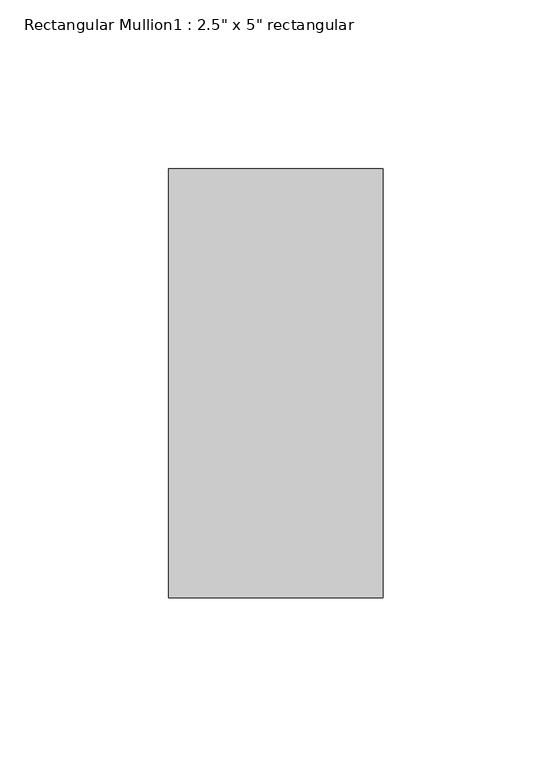
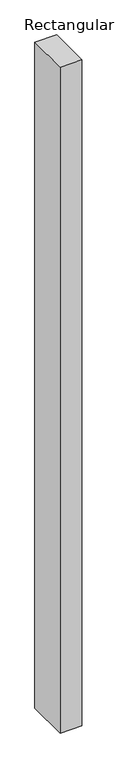
"""IFC4 building model written with IfcOpenShell, lengths in millimetres: member geometry."""

from ifc_helpers import new_model, si_unit, frame, origin, place, context, project, spatial, polyline, outline, extrude, source, transform, mapped, element, save


def member_60f5540e(model_context):
    return source(origin(), model_context, "Body", "SweptSolid", [
        extrude(outline(polyline([(0.0, 63.5), (0.0, -63.5), (-63.5, -63.5), (-63.5, 63.5), (0.0, 63.5)])), frame((0.0, 0.0, -2053.1666667), z_axis=(0.0, 0.0, 1.0), x_axis=(1.0, 0.0, 0.0)), (0.0, 0.0, 1.0), 2053.1666667),
    ])


if __name__ == "__main__":
    model = new_model("IFC4")
    model_context = context("Model", 3, world=origin())
    ifc_project = project(units=[si_unit("LENGTHUNIT", "METRE", prefix="MILLI")], contexts=[model_context])
    site = spatial("IfcSite", under=ifc_project)
    building = spatial("IfcBuilding", under=site)
    placement = place(None, origin())
    member_shape = member_60f5540e(model_context)
    element("IfcMember", 1, ObjectType="Rectangular Mullion1 : 2.5\" x 5\" rectangular", at=placement, inside=building, context=model_context, shape_type="MappedRepresentation", body=[
        mapped(member_shape, transform((0.0, 0.0, 0.0), x_axis=(1.0, 0.0, 0.0), y_axis=(0.0, 1.0, 0.0), z_axis=(0.0, 0.0, 1.0))),
    ])
    save(model, "model.ifc")

# Revit data of these elements
# Type "Rectangular Mullion1 : 2.5\" x 5\" rectangular"
#   built-in parameter 1007304 = 0.416667 (stored number, unit not read)
#   built-in parameter 1007301 = 0.104167 (stored number, unit not read)
#   built-in parameter 1007300 = 0.104167 (stored number, unit not read)
# Element 1 (IfcMember, "Rectangular Mullion1 : 2.5\" x 5\" rectangular")
#   Materials on its faces: "support-frame"
# Materials
#   "support-frame": class "Unassigned", colour RGB 233 233 233, transparency 0, Cost = 0
